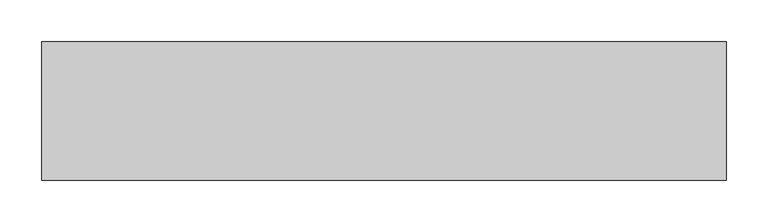
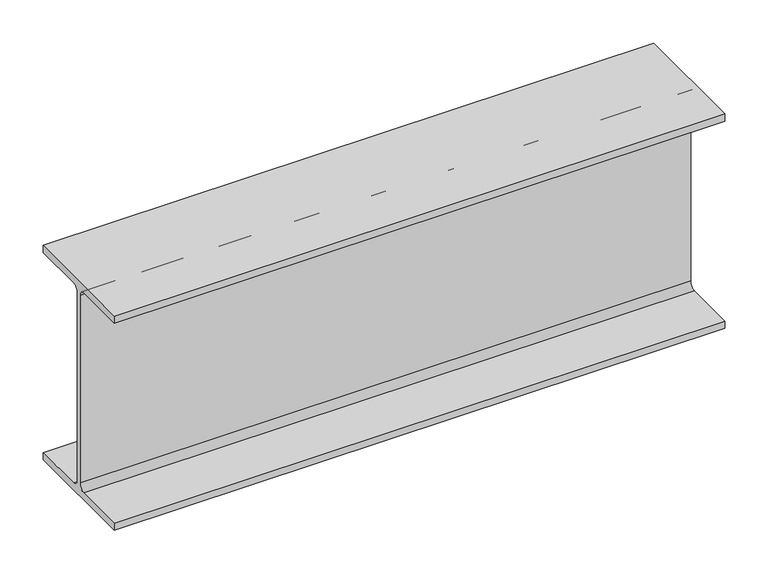
"""IFC4 building model written with IfcOpenShell, lengths in millimetres: beam geometry, Old_Steel Beam_H-KSD3502 : H_SB_ASB_H-390×300x10x16."""

from ifc_helpers import new_model, si_unit, point, frame, frame_2d, origin, place, context, project, spatial, polyline, circle_curve, trimmed, segment, composite_curve, outline, extrude, source, transform, mapped, element, save


def beam_a5681962(model_context):
    return source(origin(), model_context, "Body", "SweptSolid", [
        extrude(outline(composite_curve([segment(polyline([(82.5, -141.5), (82.5, -151.7), (-82.5, -151.7), (-82.5, -141.5), (-11.9, -141.5)]), True, "CONTINUOUS"), segment(trimmed(circle_curve(frame_2d((-11.9, -132.6)), 8.9), [point((-11.9, -141.5))], [point((-3.0, -132.6))], True, "CARTESIAN"), True, "CONTINUOUS"), segment(polyline([(-3.0, -132.6), (-3.0, 132.6)]), True, "CONTINUOUS"), segment(trimmed(circle_curve(frame_2d((-11.9, 132.6)), 8.9), [point((-3.0, 132.6))], [point((-11.9, 141.5))], True, "CARTESIAN"), True, "CONTINUOUS"), segment(polyline([(-11.9, 141.5), (-82.5, 141.5), (-82.5, 151.7), (82.5, 151.7), (82.5, 141.5), (11.9, 141.5)]), True, "CONTINUOUS"), segment(trimmed(circle_curve(frame_2d((11.9, 132.6)), 8.9), [point((11.9, 141.5))], [point((3.0, 132.6))], True, "CARTESIAN"), True, "CONTINUOUS"), segment(polyline([(3.0, 132.6), (3.0, -132.6)]), True, "CONTINUOUS"), segment(trimmed(circle_curve(frame_2d((11.9, -132.6)), 8.9), [point((3.0, -132.6))], [point((11.9, -141.5))], True, "CARTESIAN"), True, "CONTINUOUS"), segment(polyline([(11.9, -141.5), (82.5, -141.5)]), True, "CONTINUOUS")], self_intersect=False)), frame((-415.0, 0.0, 0.0), z_axis=(1.0, 0.0, 0.0), x_axis=(0.0, 1.0, 0.0)), (0.0, 0.0, 1.0), 817.2999994),
    ])


if __name__ == "__main__":
    model = new_model("IFC4")
    model_context = context("Model", 3, world=origin())
    ifc_project = project(units=[si_unit("LENGTHUNIT", "METRE", prefix="MILLI")], contexts=[model_context])
    site = spatial("IfcSite", under=ifc_project)
    building = spatial("IfcBuilding", under=site)
    placement = place(None, origin())
    beam_shape = beam_a5681962(model_context)
    element("IfcBeam", 1, ObjectType="Old_Steel Beam_H-KSD3502 : H_SB_ASB_H-390×300x10x16", at=placement, inside=building, context=model_context, shape_type="MappedRepresentation", body=[
        mapped(beam_shape, transform((0.0, 0.0, 0.0), x_axis=(1.0, 0.0, 0.0), y_axis=(0.0, 1.0, 0.0), z_axis=(0.0, 0.0, 1.0))),
    ])
    save(model, "model.ifc")

# Revit data of these elements
# Type "Old_Steel Beam_H-KSD3502 : H_SB_ASB_H-390×300x10x16"
#   Width = 30.0 cm
#   Web Thickness = 1.0 cm
#   Web Fillet = 2.2 cm
#   Warping Constant = 2517770.0 cm⁶
#   Torsional Moment of Inertia = 94.3867 cm⁴
#   Torsional Modulus = 1.0 cm³
#   Section Area = 136.0 cm²
#   Plastic Modulus weak axis = 733.0 cm³
#   Plastic Modulus strong axis = 2190.0 cm³
#   Perimeter = 1.92 m²/m
#   Nominal Weight = 107.00 kgf/m
#   Moment of Inertia weak axis = 7210.00 cm⁴
#   Moment of Inertia strong axis = 38700.00 cm⁴
#   Height = 39.0 cm
#   Flange Thickness = 1.6 cm
#   Elastic Modulus weak axis = 481.0 cm³
#   Elastic Modulus strong axis = 1980.0 cm³
#   Centroid Vertical = 19.5 cm
#   Centroid Horizontal = 15.0 cm
#   Length [instance default] = 1.5240 m
#   Structural Material [instance default] = Steel, 45-345
#   Assembly Code = ""
# Element 1 (IfcBeam, "Old_Steel Beam_H-KSD3502 : H_SB_ASB_H-390×300x10x16")
#   Structural Material = none
# Materials
#   "Steel, 45-345": class "Metal", colour RGB 189 187 185, transparency 0, Description = "Steel 345 MPa", Cost = 0
